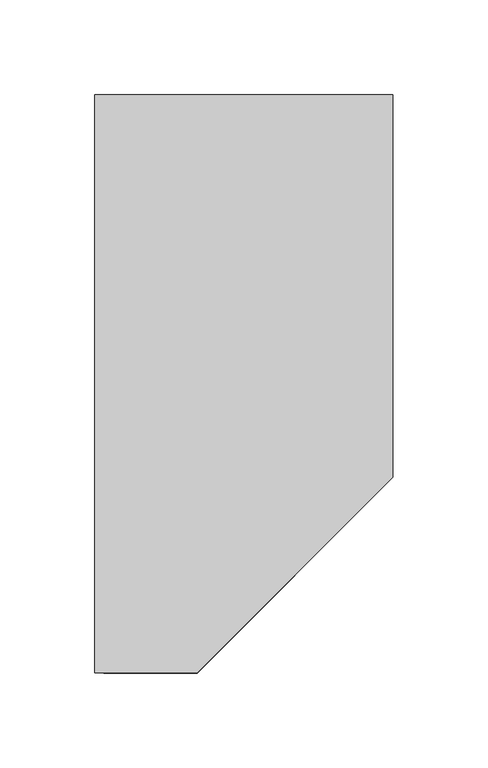
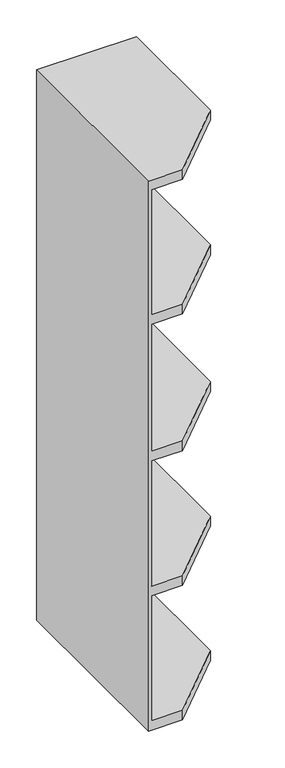
"""IFC4 building model written with IfcOpenShell, lengths in millimetres: furniture geometry, Accessories-Merillat-Wall_End_Shelf-Open : SWEOS36."""

from ifc_helpers import new_model, si_unit, origin, place, context, project, spatial, faceted_brep, source, transform, mapped, element, save


def furniture_c8c9831b(model_context):
    return source(origin(), model_context, "Body", "Brep", [
        faceted_brep([(5.0794674, -366.7125, 2133.6), (-48.8100872, -366.7125, 2133.6), (-48.8100872, -366.7125, 1219.2), (5.0794674, -366.7125, 1219.2), (5.0794674, -366.7125, 1235.075), (-44.0475872, -366.7125, 1235.075), (-44.0475872, -366.7125, 1443.0375), (5.0794674, -366.7125, 1443.0375), (5.0794674, -366.7125, 1458.9125), (-44.0475872, -366.7125, 1458.9125), (-44.0475872, -366.7125, 1666.875), (5.0794674, -366.7125, 1666.875), (5.0794674, -366.7125, 1682.75), (-44.0475872, -366.7125, 1682.75), (-44.0475872, -366.7125, 1893.8875), (5.0794674, -366.7125, 1893.8875), (5.0794674, -366.7125, 1909.7625), (-44.0475872, -366.7125, 1909.7625), (-44.0475872, -366.7125, 2117.725), (5.0794674, -366.7125, 2117.725), (-44.0475872, -66.9237697, 1682.75), (-44.0475872, -66.9237697, 1893.8875), (-44.0475872, -66.9237697, 1235.075), (-44.0475872, -66.9237697, 1443.0375), (-44.0475872, -66.9237697, 1458.9125), (-44.0475872, -66.9237697, 1666.875), (-44.0475872, -66.9237697, 1909.7625), (-44.0475872, -66.9237697, 2117.725), (108.3524128, -263.4395546, 1682.75), (108.3524128, -66.9237697, 1682.75), (108.3524128, -263.4395546, 1666.875), (108.3524128, -66.9237697, 1666.875), (108.3524128, -263.4395546, 1458.9125), (108.3524128, -66.9237697, 1458.9125), (108.3524128, -263.4395546, 1443.0375), (108.3524128, -66.9237697, 1443.0375), (108.3524128, -263.4395546, 1235.075), (108.3524128, -66.9237697, 1235.075), (108.3524128, -263.4395546, 1219.2), (-48.8100872, -61.9125, 1219.2), (108.3524128, -61.9125, 1219.2), (-48.8100872, -61.9125, 2133.6), (-48.8100872, -61.9125, 1682.75), (-48.8100872, -61.9125, 1666.875), (108.3524128, -61.9125, 2133.6), (108.3524128, -263.4395546, 2117.725), (108.3524128, -66.9237697, 2117.725), (108.3524128, -66.9237697, 1909.7625), (108.3524128, -263.4395546, 1909.7625), (108.3524128, -263.4395546, 1893.8875), (108.3524128, -66.9237697, 1893.8875), (108.3524128, -263.4395546, 2133.6)], [[[0, 1, 2, 3, 4, 5, 6, 7, 8, 9, 10, 11, 12, 13, 14, 15, 16, 17, 18, 19]], [[14, 13, 20, 21]], [[5, 22, 23, 6]], [[24, 25, 10, 9]], [[17, 26, 27, 18]], [[28, 29, 20, 13, 12]], [[12, 11, 30, 28]], [[11, 10, 25, 31, 30]], [[32, 33, 24, 9, 8]], [[8, 7, 34, 32]], [[7, 6, 23, 35, 34]], [[36, 37, 22, 5, 4]], [[4, 3, 38, 36]], [[39, 40, 38, 3, 2]], [[41, 42, 43, 39, 2, 1]], [[40, 39, 43, 42, 41, 44]], [[45, 46, 47, 48, 49, 50, 29, 28, 30, 31, 33, 32, 34, 35, 37, 36, 38, 40, 44, 51]], [[21, 20, 29, 50]], [[35, 23, 22, 37]], [[33, 31, 25, 24]], [[46, 27, 26, 47]], [[51, 44, 41, 1, 0]], [[19, 18, 27, 46, 45]], [[0, 19, 45, 51]], [[48, 47, 26, 17, 16]], [[15, 14, 21, 50, 49]], [[16, 15, 49, 48]]]),
    ])


if __name__ == "__main__":
    model = new_model("IFC4")
    model_context = context("Model", 3, world=origin())
    ifc_project = project(units=[si_unit("LENGTHUNIT", "METRE", prefix="MILLI")], contexts=[model_context])
    site = spatial("IfcSite", under=ifc_project)
    building = spatial("IfcBuilding", under=site)
    placement = place(None, origin())
    furniture_shape = furniture_c8c9831b(model_context)
    element("IfcFurniture", 1, ObjectType="Accessories-Merillat-Wall_End_Shelf-Open : SWEOS36", at=placement, inside=building, context=model_context, shape_type="MappedRepresentation", body=[
        mapped(furniture_shape, transform((0.0, 0.0, 0.0), x_axis=(1.0, 0.0, 0.0), y_axis=(0.0, 1.0, 0.0), z_axis=(0.0, 0.0, 1.0))),
    ])
    save(model, "model.ifc")

# Revit data of these elements
# Type "Accessories-Merillat-Wall_End_Shelf-Open : SWEOS36"
#   URL = "https://www.merillat.com/"
#   Product Page URL = "https://www.merillat.com/our-products/rooms/kitchen/"
#   Product Documentation Link = "http://merillatbusiness.com/wp-content/uploads/2014/07/Merillat_Classic_Catalog.pdf"
#   Model = "SWEOS36"
#   Manufacturer = "Merillat"
#   Finish = "Wood"
#   Description = "Solid Wood Wall End Open Shelf 36"
#   Construction Type = "Wall Cabinet"
#   Cabinet Construction Note = "Trimmable to 5 7/8 inches wide, Invertible for right or left hand use"
#   Assembly Code = "C1030410"
#   Shelf Thickness = 0' - 0 5/8"
#   Shelf Spacing = 0' - 8 3/16"
#   Depth = 1' - 0"
#   Height = 3' - 0"
#   Top Of Cabinet = 7' - 0"
#   Width = 0' - 6 3/16"
#   COBie.Type = no
#   Fourth Shelf = yes
#   Cabinet Material = Wood - Merillat - Pecan(1)
# Element 1 (IfcFurniture, "Accessories-Merillat-Wall_End_Shelf-Open : SWEOS36")
#   Materials on its faces: "Wood - Merillat - Pecan(1)"
# Materials
#   "Wood - Merillat - Pecan(1)": class "Wood", colour RGB 108 67 43, transparency 0, Cost = 0
